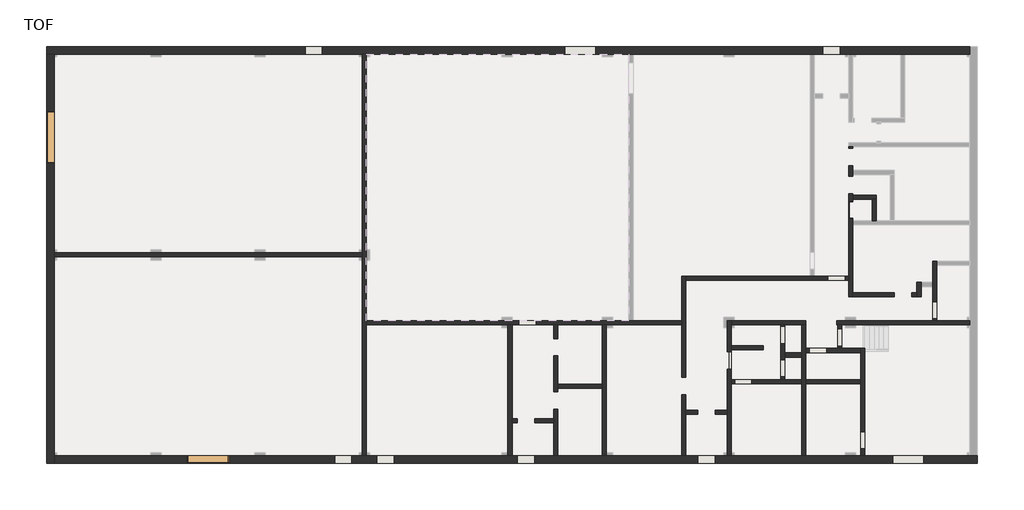
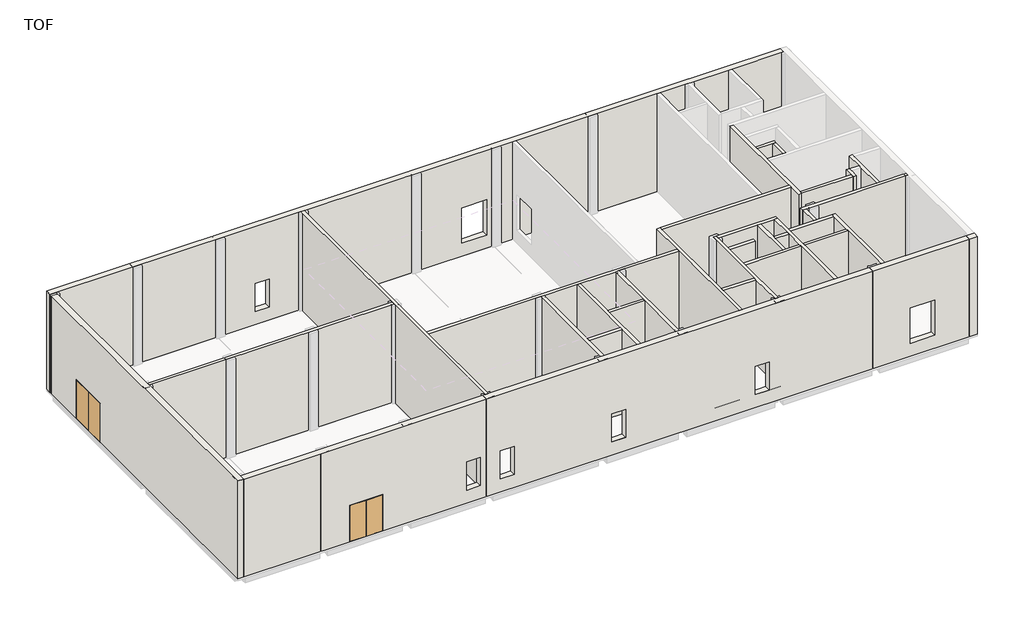
# One storey, part 1 of 3: 31 walls, 3 doors.
# Revit data of these elements (continued)
# Grids (mm) (continued)
#   "Y1": line (-3935.398, 24016.521) -> (58968.688, 24016.521)
#   "X1": line (-75.3, 29394.337) -> (-75.3, -4379.638)
#   "X2": line (5924.7, 29394.337) -> (5924.7, -4379.638)
#   "Y3": line (-3935.398, 8416.521) -> (58968.688, 8416.521)
#   "Y4": line (-3935.398, 616.521) -> (58968.688, 616.521)
#   "X3": line (11924.7, 29394.337) -> (11924.7, -4379.638)
#   "X4": line (17924.7, 29394.337) -> (17924.7, -4379.638)
#   "X5": line (26124.7, 29394.337) -> (26124.7, -4379.638)
#   "X6": line (31924.7, 29394.337) -> (31924.7, -4379.638)
#   "X7": line (38924.7, 29394.337) -> (38924.7, -4379.638)
#   "X8": line (45924.7, 29394.337) -> (45924.7, -4379.638)
#   "X9": line (52924.7, 29394.337) -> (52924.7, -4379.638)
#   "X15": line (43724.7, 27041.858) -> (43724.7, 9156.488)
#   "X16": line (36324.7, 27041.858) -> (36324.7, 9156.488)
#   "X17": line (34685.051, 10966.521) -> (55094.626, 10966.521)
#   "X18": line (34685.051, 18666.521) -> (55094.626, 18666.521)
#   "Y2": line (-3935.398, 12316.521) -> (58968.688, 12316.521)
# Type "Double Door_Steel : H_DR_AMB_Double Door_Steel_W3000xH3000"
#   Type Mark = "362"
#   프레임 = ""
#   철물 = ""
#   유리/마감 = ""
#   위치/개소 = ""
#   부호 = "1/SD"
#   문번호 = ""
#   문기호 = "SD"
#   Analytic Construction = "<None>"
#   Height = 3000.000 mm
#   Width = 3000.000 mm
#   Define Thermal Properties by = 1
#   문 틀 = none
#   문 = none
#   Function = (empty or 0)
#   Assembly Code = ""
#   Wall Closure = (empty or 0)
# Type "Double Door_Steel : H_DR_AMB_Double Door_Steel_W2400xH2800"
#   Type Mark = "365"
#   프레임 = ""
#   철물 = ""
#   유리/마감 = ""
#   위치/개소 = ""
#   부호 = "1/SD"
#   문번호 = ""
#   문기호 = "SD"
#   Analytic Construction = "<None>"
#   Height = 2800.000 mm
#   Width = 2400.000 mm
#   Define Thermal Properties by = 1
#   문 틀 = none
#   문 = none
#   Function = (empty or 0)
#   Assembly Code = ""
#   Wall Closure = (empty or 0)
# Type "Double Door_Steel : H_DR_AMB_Double Door_Steel_W1000xH2150"
#   Type Mark = "366"
#   프레임 = ""
#   철물 = ""
#   유리/마감 = ""
#   위치/개소 = ""
#   부호 = "1/SD"
#   문번호 = ""
#   문기호 = "SD"
#   Analytic Construction = "<None>"
#   Height = 2150.000 mm
#   Width = 1000.000 mm
#   Define Thermal Properties by = 1
#   문 틀 = none
#   문 = none
#   Function = (empty or 0)
#   Assembly Code = ""
#   Wall Closure = (empty or 0)
# Type "H_WA_AMW_Brick Wall_Ext (0.5B_50_1.0B / Emulsion)"
#   Type Comments = ""
#   Layers, outside or top first: 0.000 mm no material (function 100); 20.000 mm no material (function 2); 115.000 mm no material (function 1); 50.000 mm no material (function 3); 0.000 mm no material (function 100); 230.000 mm no material (function 1); 15.000 mm no material (function 2); 0.000 mm no material (function 100); 0.000 mm no material (function 100)
# Type "H_WA_AMW_Block Wall_Int_T200 (Both Plaster_Emulsion)"
#   Type Comments = ""
#   Layers, outside or top first: 0.000 mm no material (function 100); 12.000 mm no material (function 2); 200.000 mm no material (function 1); 12.000 mm no material (function 2); 10.000 mm no material (function 5)
# Element 1 (IfcDoor, "Double Door_Steel : H_DR_AMB_Double Door_Steel_W3000xH3000")
#   Phase Created = New Construction
# Element 2 (IfcDoor, "Double Door_Steel : H_DR_AMB_Double Door_Steel_W2400xH2800")
#   Phase Created = New Construction
# Element 3 (IfcDoor, "Double Door_Steel : H_DR_AMB_Double Door_Steel_W1000xH2150")
#   Phase Created = New Construction
# Element 4 (IfcWall, "H_WA_AMW_Brick Wall_Ext (0.5B_50_1.0B / Emulsion)")
#   Mark = "EW1"
#   Wall Loca = "EXT"
#   Wall Style Name = "Concrete Wall+Insulation+Gypsum Board"
#   Wall Finish-In = "Acrylic Emulsion Paint on Gypsum Board"
#   Wall Base Material-2 = "Glass Wool (Fiberglass)"
#   Wall Base Material-3 = "Concrete Wall"
#   Wall Finish-Ex = "Acrylic Emulsion Paint on Fair Faced Concrete"
#   Top Offset = 0.000 mm
#   Base Offset = 0.000 mm
#   wall height = 7500.000 mm
#   Wall Style No = EW51-1
#   Phase Created = New Construction
#   Base Constraint = TOF
#   Top Constraint = TOC
#   Materials on its faces: "Default Wall"
# Element 5 (IfcWall, "H_WA_AMW_Brick Wall_Ext (0.5B_50_1.0B / Emulsion)")
#   Mark = "EW2"
#   Wall Loca = "EXT"
#   Wall Style Name = "Concrete Wall+Insulation+Gypsum Board"
#   Wall Finish-In = "Acrylic Emulsion Paint on Gypsum Board"
#   Wall Base Material-2 = "Glass Wool (Fiberglass)"
#   Wall Base Material-3 = "Concrete Wall"
#   Wall Finish-Ex = "Acrylic Emulsion Paint on Fair Faced Concrete"
#   Top Offset = 0.000 mm
#   Base Offset = 0.000 mm
#   wall height = 7500.000 mm
#   Wall Style No = EW51-1
#   Phase Created = New Construction
#   Base Constraint = TOF
#   Top Constraint = TOC
#   Materials on its faces: "Default Wall"
# Element 6 (IfcWall, "H_WA_AMW_Brick Wall_Ext (0.5B_50_1.0B / Emulsion)")
#   Mark = "EW3"
#   Wall Loca = "EXT"
#   Wall Style Name = "Concrete Wall+Insulation+Gypsum Board"
#   Wall Finish-In = "Acrylic Emulsion Paint on Gypsum Board"
#   Wall Base Material-2 = "Glass Wool (Fiberglass)"
#   Wall Base Material-3 = "Concrete Wall"
#   Wall Finish-Ex = "Acrylic Emulsion Paint on Fair Faced Concrete"
#   Top Offset = 0.000 mm
#   Base Offset = 0.000 mm
#   wall height = 7500.000 mm
#   Wall Style No = EW51-1
#   Phase Created = New Construction
#   Base Constraint = TOF
#   Top Constraint = TOC
#   Materials on its faces: "Default Wall"
# Element 7 (IfcWall, "H_WA_AMW_Block Wall_Int_T200 (Both Plaster_Emulsion)")
#   Mark = "W1"
#   Wall Loca = "INT"
#   Wall Style Name = "Block Wall"
#   Wall Ref. = ""
#   Wall Finish-In = "Acrylic Emulsion Paint on Cement Plaster"
#   Wall Base Material-1 = "Concrete Block"
#   Wall Base Material-2 = ""
#   Wall Base Material-3 = ""
#   Wall Finish-Ex = "Acrylic Emulsion Paint on Cement Plaster"
#   Top Offset = 0.000 mm
#   Base Offset = 0.000 mm
#   wall height = 7500.000 mm
#   Wall Style No = IW21
#   Phase Created = New Construction
#   Base Constraint = TOF
#   Top Constraint = TOC
#   Materials on its faces: "Default Wall"
# Element 8 (IfcWall, "H_WA_AMW_Block Wall_Int_T200 (Both Plaster_Emulsion)")
#   Mark = "W2"
#   Wall Loca = "INT"
#   Wall Style Name = "Block Wall"
#   Wall Ref. = ""
#   Wall Finish-In = "Acrylic Emulsion Paint on Cement Plaster"
#   Wall Base Material-1 = "Concrete Block"
#   Wall Base Material-2 = ""
#   Wall Base Material-3 = ""
#   Wall Finish-Ex = "Acrylic Emulsion Paint on Cement Plaster"
#   Top Offset = 0.000 mm
#   Base Offset = 0.000 mm
#   wall height = 7500.000 mm
#   Wall Style No = IW21
#   Phase Created = New Construction
#   Base Constraint = TOF
#   Top Constraint = TOC
#   Materials on its faces: "Default Wall"
# Element 9 (IfcWall, "H_WA_AMW_Block Wall_Int_T200 (Both Plaster_Emulsion)")
#   Mark = "W4"
#   Wall Loca = "INT"
#   Wall Style Name = "Block Wall"
#   Wall Ref. = ""
#   Wall Finish-In = "Acrylic Emulsion Paint on Cement Plaster"
#   Wall Base Material-1 = "Concrete Block"
#   Wall Base Material-2 = ""
#   Wall Base Material-3 = ""
#   Wall Finish-Ex = "Acrylic Emulsion Paint on Cement Plaster"
#   Top Offset = 0.000 mm
#   Base Offset = 0.000 mm
#   wall height = 7500.000 mm
#   Wall Style No = IW21
#   Phase Created = New Construction
#   Base Constraint = TOF
#   Top Constraint = TOC
#   Materials on its faces: "Default Wall"
# Element 10 (IfcWall, "H_WA_AMW_Block Wall_Int_T200 (Both Plaster_Emulsion)")
#   Mark = "W5"
#   Wall Loca = "INT"
#   Wall Style Name = "Block Wall"
#   Wall Ref. = ""
#   Wall Finish-In = "Acrylic Emulsion Paint on Cement Plaster"
#   Wall Base Material-1 = "Concrete Block"
#   Wall Base Material-2 = ""
#   Wall Base Material-3 = ""
#   Wall Finish-Ex = "Acrylic Emulsion Paint on Cement Plaster"
#   built-in parameter 1001111 = 1000.000 mm
#   Top Offset = 0.000 mm
#   Base Offset = 1000.000 mm
#   wall height = 6500.000 mm
#   Wall Style No = IW21
#   Phase Created = New Construction
#   Base Constraint = TOF
#   Top Constraint = TOC
#   Materials on its faces: "Default Wall"
# Element 11 (IfcWall, "H_WA_AMW_Block Wall_Int_T200 (Both Plaster_Emulsion)")
#   Mark = "W6"
#   Wall Loca = "INT"
#   Wall Style Name = "Block Wall"
#   Wall Ref. = ""
#   Wall Finish-In = "Acrylic Emulsion Paint on Cement Plaster"
#   Wall Base Material-1 = "Concrete Block"
#   Wall Base Material-2 = ""
#   Wall Base Material-3 = ""
#   Wall Finish-Ex = "Acrylic Emulsion Paint on Cement Plaster"
#   Top Offset = 0.000 mm
#   Base Offset = 0.000 mm
#   wall height = 7500.000 mm
#   Wall Style No = IW21
#   Phase Created = New Construction
#   Base Constraint = TOF
#   Top Constraint = TOC
#   Materials on its faces: "Default Wall"
# Element 12 (IfcWall, "H_WA_AMW_Block Wall_Int_T200 (Both Plaster_Emulsion)")
#   Mark = "W10"
#   Wall Loca = "INT"
#   Wall Style Name = "Block Wall"
#   Wall Ref. = ""
#   Wall Finish-In = "Acrylic Emulsion Paint on Cement Plaster"
#   Wall Base Material-1 = "Concrete Block"
#   Wall Base Material-2 = ""
#   Wall Base Material-3 = ""
#   Wall Finish-Ex = "Acrylic Emulsion Paint on Cement Plaster"
#   built-in parameter 1001111 = 1000.000 mm
#   Top Offset = 0.000 mm
#   Base Offset = 1000.000 mm
#   wall height = 6500.000 mm
#   Wall Style No = IW21
#   Phase Created = New Construction
#   Base Constraint = TOF
#   Top Constraint = TOC
#   Materials on its faces: "Default Wall"
# Element 13 (IfcWall, "H_WA_AMW_Block Wall_Int_T200 (Both Plaster_Emulsion)")
#   Mark = "W11"
#   Wall Loca = "INT"
#   Wall Style Name = "Block Wall"
#   Wall Ref. = ""
#   Wall Finish-In = "Acrylic Emulsion Paint on Cement Plaster"
#   Wall Base Material-1 = "Concrete Block"
#   Wall Base Material-2 = ""
#   Wall Base Material-3 = ""
#   Wall Finish-Ex = "Acrylic Emulsion Paint on Cement Plaster"
#   Top Offset = 0.000 mm
#   Base Offset = 0.000 mm
#   wall height = 7500.000 mm
#   Wall Style No = IW21
#   Phase Created = New Construction
#   Base Constraint = TOF
#   Top Constraint = TOC
#   Materials on its faces: "Default Wall"
# Element 14 (IfcWall, "H_WA_AMW_Block Wall_Int_T200 (Both Plaster_Emulsion)")
#   Mark = "W13"
#   Wall Loca = "INT"
#   Wall Style Name = "Block Wall"
#   Wall Ref. = ""
#   Wall Finish-In = "Acrylic Emulsion Paint on Cement Plaster"
#   Wall Base Material-1 = "Concrete Block"
#   Wall Base Material-2 = ""
#   Wall Base Material-3 = ""
#   Wall Finish-Ex = "Acrylic Emulsion Paint on Cement Plaster"
#   built-in parameter 1001111 = 1000.000 mm
#   Top Offset = 0.000 mm
#   Base Offset = 1000.000 mm
#   wall height = 6500.000 mm
#   Wall Style No = IW21
#   Phase Created = New Construction
#   Base Constraint = TOF
#   Top Constraint = TOC
#   Materials on its faces: "Default Wall"
# Element 15 (IfcWall, "H_WA_AMW_Block Wall_Int_T200 (Both Plaster_Emulsion)")
#   Mark = "W15"
#   Wall Loca = "INT"
#   Wall Style Name = "Block Wall"
#   Wall Ref. = ""
#   Wall Finish-In = "Acrylic Emulsion Paint on Cement Plaster"
#   Wall Base Material-1 = "Concrete Block"
#   Wall Base Material-2 = ""
#   Wall Base Material-3 = ""
#   Wall Finish-Ex = "Acrylic Emulsion Paint on Cement Plaster"
#   Top Offset = 0.000 mm
#   Base Offset = 0.000 mm
#   wall height = 7500.000 mm
#   Wall Style No = IW21
#   Phase Created = New Construction
#   Base Constraint = TOF
#   Top Constraint = TOC
#   Materials on its faces: "Default Wall"
# Element 16 (IfcWall, "H_WA_AMW_Block Wall_Int_T200 (Both Plaster_Emulsion)")
#   Mark = "W16"
#   Wall Loca = "INT"
#   Wall Style Name = "Block Wall"
#   Wall Ref. = ""
#   Wall Finish-In = "Acrylic Emulsion Paint on Cement Plaster"
#   Wall Base Material-1 = "Concrete Block"
#   Wall Base Material-2 = ""
#   Wall Base Material-3 = ""
#   Wall Finish-Ex = "Acrylic Emulsion Paint on Cement Plaster"
#   Top Offset = 0.000 mm
#   Base Offset = 0.000 mm
#   wall height = 7500.000 mm
#   Wall Style No = IW21
#   Phase Created = New Construction
#   Base Constraint = TOF
#   Top Constraint = TOC
#   Materials on its faces: "Default Wall"
# Element 17 (IfcWall, "H_WA_AMW_Block Wall_Int_T200 (Both Plaster_Emulsion)")
#   Mark = "W17"
#   Wall Loca = "INT"
#   Wall Style Name = "Block Wall"
#   Wall Ref. = ""
#   Wall Finish-In = "Acrylic Emulsion Paint on Cement Plaster"
#   Wall Base Material-1 = "Concrete Block"
#   Wall Base Material-2 = ""
#   Wall Base Material-3 = ""
#   Wall Finish-Ex = "Acrylic Emulsion Paint on Cement Plaster"
#   Top Offset = 0.000 mm
#   Base Offset = 0.000 mm
#   wall height = 7500.000 mm
#   Wall Style No = IW21
#   Phase Created = New Construction
#   Base Constraint = TOF
#   Top Constraint = TOC
#   Materials on its faces: "Default Wall"
# Element 18 (IfcWall, "H_WA_AMW_Block Wall_Int_T200 (Both Plaster_Emulsion)")
#   Mark = "W18"
#   Wall Loca = "INT"
#   Wall Style Name = "Block Wall"
#   Wall Ref. = ""
#   Wall Finish-In = "Acrylic Emulsion Paint on Cement Plaster"
#   Wall Base Material-1 = "Concrete Block"
#   Wall Base Material-2 = ""
#   Wall Base Material-3 = ""
#   Wall Finish-Ex = "Acrylic Emulsion Paint on Cement Plaster"
#   Top Offset = 0.000 mm
#   Base Offset = 0.000 mm
#   wall height = 7500.000 mm
#   Wall Style No = IW21
#   Phase Created = New Construction
#   Base Constraint = TOF
#   Top Constraint = TOC
#   Materials on its faces: "Default Wall"
# Element 19 (IfcWall, "H_WA_AMW_Block Wall_Int_T200 (Both Plaster_Emulsion)")
#   Mark = "W19"
#   Wall Loca = "INT"
#   Wall Style Name = "Block Wall"
#   Wall Ref. = ""
#   Wall Finish-In = "Acrylic Emulsion Paint on Cement Plaster"
#   Wall Base Material-1 = "Concrete Block"
#   Wall Base Material-2 = ""
#   Wall Base Material-3 = ""
#   Wall Finish-Ex = "Acrylic Emulsion Paint on Cement Plaster"
#   Top Offset = 0.000 mm
#   Base Offset = 0.000 mm
#   wall height = 7500.000 mm
#   Wall Style No = IW21
#   Phase Created = New Construction
#   Base Constraint = TOF
#   Top Constraint = TOC
#   Materials on its faces: "Default Wall"
# Element 20 (IfcWall, "H_WA_AMW_Block Wall_Int_T200 (Both Plaster_Emulsion)")
#   Mark = "W20"
#   Wall Loca = "INT"
#   Wall Style Name = "Block Wall"
#   Wall Ref. = ""
#   Wall Finish-In = "Acrylic Emulsion Paint on Cement Plaster"
#   Wall Base Material-1 = "Concrete Block"
#   Wall Base Material-2 = ""
#   Wall Base Material-3 = ""
#   Wall Finish-Ex = "Acrylic Emulsion Paint on Cement Plaster"
#   Top Offset = 0.000 mm
#   Base Offset = 0.000 mm
#   wall height = 7500.000 mm
#   Wall Style No = IW21
#   Phase Created = New Construction
#   Base Constraint = TOF
#   Top Constraint = TOC
#   Materials on its faces: "Default Wall"
# Element 21 (IfcWall, "H_WA_AMW_Block Wall_Int_T200 (Both Plaster_Emulsion)")
#   Mark = "W21"
#   Wall Loca = "INT"
#   Wall Style Name = "Block Wall"
#   Wall Ref. = ""
#   Wall Finish-In = "Acrylic Emulsion Paint on Cement Plaster"
#   Wall Base Material-1 = "Concrete Block"
#   Wall Base Material-2 = ""
#   Wall Base Material-3 = ""
#   Wall Finish-Ex = "Acrylic Emulsion Paint on Cement Plaster"
#   Top Offset = 0.000 mm
#   Base Offset = 0.000 mm
#   wall height = 7500.000 mm
#   Wall Style No = IW21
#   Phase Created = New Construction
#   Base Constraint = TOF
#   Top Constraint = TOC
#   Materials on its faces: "Default Wall"
# Element 22 (IfcWall, "H_WA_AMW_Block Wall_Int_T200 (Both Plaster_Emulsion)")
#   Mark = "W22"
#   Wall Loca = "INT"
#   Wall Style Name = "Block Wall"
#   Wall Ref. = ""
#   Wall Finish-In = "Acrylic Emulsion Paint on Cement Plaster"
#   Wall Base Material-1 = "Concrete Block"
#   Wall Base Material-2 = ""
#   Wall Base Material-3 = ""
#   Wall Finish-Ex = "Acrylic Emulsion Paint on Cement Plaster"
#   Top Offset = 0.000 mm
#   Base Offset = 0.000 mm
#   wall height = 7500.000 mm
#   Wall Style No = IW21
#   Phase Created = New Construction
#   Base Constraint = TOF
#   Top Constraint = TOC
#   Materials on its faces: "Default Wall"
# Element 23 (IfcWall, "H_WA_AMW_Block Wall_Int_T200 (Both Plaster_Emulsion)")
#   Mark = "W23"
#   Wall Loca = "INT"
#   Wall Style Name = "Block Wall"
#   Wall Ref. = ""
#   Wall Finish-In = "Acrylic Emulsion Paint on Cement Plaster"
#   Wall Base Material-1 = "Concrete Block"
#   Wall Base Material-2 = ""
#   Wall Base Material-3 = ""
#   Wall Finish-Ex = "Acrylic Emulsion Paint on Cement Plaster"
#   Top Offset = 0.000 mm
#   Base Offset = 0.000 mm
#   wall height = 7500.000 mm
#   Wall Style No = IW21
#   Phase Created = New Construction
#   Base Constraint = TOF
#   Top Constraint = TOC
#   Materials on its faces: "Default Wall"
# Element 24 (IfcWall, "H_WA_AMW_Block Wall_Int_T200 (Both Plaster_Emulsion)")
#   Mark = "W24"
#   Wall Loca = "INT"
#   Wall Style Name = "Block Wall"
#   Wall Ref. = ""
#   Wall Finish-In = "Acrylic Emulsion Paint on Cement Plaster"
#   Wall Base Material-1 = "Concrete Block"
#   Wall Base Material-2 = ""
#   Wall Base Material-3 = ""
#   Wall Finish-Ex = "Acrylic Emulsion Paint on Cement Plaster"
#   Top Offset = 0.000 mm
#   Base Offset = 0.000 mm
#   wall height = 7500.000 mm
#   Wall Style No = IW21
#   Phase Created = New Construction
#   Base Constraint = TOF
#   Top Constraint = TOC
#   Materials on its faces: "Default Wall"
# Element 25 (IfcWall, "H_WA_AMW_Block Wall_Int_T200 (Both Plaster_Emulsion)")
#   Mark = "W25"
#   Wall Loca = "INT"
#   Wall Style Name = "Block Wall"
#   Wall Ref. = ""
#   Wall Finish-In = "Acrylic Emulsion Paint on Cement Plaster"
#   Wall Base Material-1 = "Concrete Block"
#   Wall Base Material-2 = ""
#   Wall Base Material-3 = ""
#   Wall Finish-Ex = "Acrylic Emulsion Paint on Cement Plaster"
#   built-in parameter 1001111 = 1000.000 mm
#   Top Offset = 0.000 mm
#   Base Offset = 1000.000 mm
#   wall height = 6500.000 mm
#   Wall Style No = IW21
#   Phase Created = New Construction
#   Base Constraint = TOF
#   Top Constraint = TOC
#   Materials on its faces: "Default Wall"
# Element 26 (IfcWall, "H_WA_AMW_Block Wall_Int_T200 (Both Plaster_Emulsion)")
#   Mark = "W26"
#   Wall Loca = "INT"
#   Wall Style Name = "Block Wall"
#   Wall Ref. = ""
#   Wall Finish-In = "Acrylic Emulsion Paint on Cement Plaster"
#   Wall Base Material-1 = "Concrete Block"
#   Wall Base Material-2 = ""
#   Wall Base Material-3 = ""
#   Wall Finish-Ex = "Acrylic Emulsion Paint on Cement Plaster"
#   built-in parameter 1001111 = 1000.000 mm
#   Top Offset = 0.000 mm
#   Base Offset = 1000.000 mm
#   wall height = 6500.000 mm
#   Wall Style No = IW21
#   Phase Created = New Construction
#   Base Constraint = TOF
#   Top Constraint = TOC
#   Materials on its faces: "Default Wall"
# Element 27 (IfcWall, "H_WA_AMW_Block Wall_Int_T200 (Both Plaster_Emulsion)")
#   Mark = "W27"
#   Wall Loca = "INT"
#   Wall Style Name = "Block Wall"
#   Wall Ref. = ""
#   Wall Finish-In = "Acrylic Emulsion Paint on Cement Plaster"
#   Wall Base Material-1 = "Concrete Block"
#   Wall Base Material-2 = ""
#   Wall Base Material-3 = ""
#   Wall Finish-Ex = "Acrylic Emulsion Paint on Cement Plaster"
#   Top Offset = 0.000 mm
#   Base Offset = 0.000 mm
#   wall height = 7500.000 mm
#   Wall Style No = IW21
#   Phase Created = New Construction
#   Base Constraint = TOF
#   Top Constraint = TOC
#   Materials on its faces: "Default Wall"
# Element 28 (IfcWall, "H_WA_AMW_Block Wall_Int_T200 (Both Plaster_Emulsion)")
#   Mark = "W28"
#   Wall Loca = "INT"
#   Wall Style Name = "Block Wall"
#   Wall Ref. = ""
#   Wall Finish-In = "Acrylic Emulsion Paint on Cement Plaster"
#   Wall Base Material-1 = "Concrete Block"
#   Wall Base Material-2 = ""
#   Wall Base Material-3 = ""
#   Wall Finish-Ex = "Acrylic Emulsion Paint on Cement Plaster"
#   built-in parameter 1001111 = 1000.000 mm
#   Top Offset = 0.000 mm
#   Base Offset = 1000.000 mm
#   wall height = 6500.000 mm
#   Wall Style No = IW21
#   Phase Created = New Construction
#   Base Constraint = TOF
#   Top Constraint = TOC
#   Materials on its faces: "Default Wall"
# Element 29 (IfcWall, "H_WA_AMW_Block Wall_Int_T200 (Both Plaster_Emulsion)")
#   Mark = "W29"
#   Wall Loca = "INT"
#   Wall Style Name = "Block Wall"
#   Wall Ref. = ""
#   Wall Finish-In = "Acrylic Emulsion Paint on Cement Plaster"
#   Wall Base Material-1 = "Concrete Block"
#   Wall Base Material-2 = ""
#   Wall Base Material-3 = ""
#   Wall Finish-Ex = "Acrylic Emulsion Paint on Cement Plaster"
#   built-in parameter 1001111 = 1000.000 mm
#   Top Offset = 0.000 mm
#   Base Offset = 1000.000 mm
#   wall height = 6500.000 mm
#   Wall Style No = IW21
#   Phase Created = New Construction
#   Base Constraint = TOF
#   Top Constraint = TOC
#   Materials on its faces: "Default Wall"
# Element 30 (IfcWall, "H_WA_AMW_Block Wall_Int_T200 (Both Plaster_Emulsion)")
#   Mark = "W31"
#   Wall Loca = "INT"
#   Wall Style Name = "Block Wall"
#   Wall Ref. = ""
#   Wall Finish-In = "Acrylic Emulsion Paint on Cement Plaster"
#   Wall Base Material-1 = "Concrete Block"
#   Wall Base Material-2 = ""
#   Wall Base Material-3 = ""
#   Wall Finish-Ex = "Acrylic Emulsion Paint on Cement Plaster"
#   built-in parameter 1001111 = 1000.000 mm
#   Top Offset = 0.000 mm
#   Base Offset = 1000.000 mm
#   wall height = 6500.000 mm
#   Wall Style No = IW21
#   Phase Created = New Construction
#   Base Constraint = TOF
#   Top Constraint = TOC
#   Materials on its faces: "Default Wall"
# Element 31 (IfcWall, "H_WA_AMW_Block Wall_Int_T200 (Both Plaster_Emulsion)")
#   Mark = "W34"
#   Wall Loca = "INT"
#   Wall Style Name = "Block Wall"
#   Wall Ref. = ""
#   Wall Finish-In = "Acrylic Emulsion Paint on Cement Plaster"
#   Wall Base Material-1 = "Concrete Block"
#   Wall Base Material-2 = ""
#   Wall Base Material-3 = ""
#   Wall Finish-Ex = "Acrylic Emulsion Paint on Cement Plaster"
#   built-in parameter 1001111 = 1000.000 mm
#   Top Offset = 0.000 mm
#   Base Offset = 1000.000 mm
#   wall height = 6500.000 mm
#   Wall Style No = IW21
#   Phase Created = New Construction
#   Base Constraint = TOF
#   Top Constraint = TOC
#   Materials on its faces: "Default Wall"
# Element 32 (IfcWall, "H_WA_AMW_Block Wall_Int_T200 (Both Plaster_Emulsion)")
#   Mark = "W39"
#   Wall Loca = "INT"
#   Wall Style Name = "Block Wall"
#   Wall Ref. = ""
#   Wall Finish-In = "Acrylic Emulsion Paint on Cement Plaster"
#   Wall Base Material-1 = "Concrete Block"
#   Wall Base Material-2 = ""
#   Wall Base Material-3 = ""
#   Wall Finish-Ex = "Acrylic Emulsion Paint on Cement Plaster"
#   built-in parameter 1001111 = 1000.000 mm
#   Top Offset = 0.000 mm
#   Base Offset = 1000.000 mm
#   wall height = 6500.000 mm
#   Wall Style No = IW21
#   Phase Created = New Construction
#   Base Constraint = TOF
#   Top Constraint = TOC
#   Materials on its faces: "Default Wall"
# Element 33 (IfcWall, "H_WA_AMW_Block Wall_Int_T200 (Both Plaster_Emulsion)")
#   Mark = "W40"
#   Wall Loca = "INT"
#   Wall Style Name = "Block Wall"
#   Wall Ref. = ""
#   Wall Finish-In = "Acrylic Emulsion Paint on Cement Plaster"
#   Wall Base Material-1 = "Concrete Block"
#   Wall Base Material-2 = ""
#   Wall Base Material-3 = ""
#   Wall Finish-Ex = "Acrylic Emulsion Paint on Cement Plaster"
#   built-in parameter 1001111 = 1000.000 mm
#   Top Offset = 0.000 mm
#   Base Offset = 1000.000 mm
#   wall height = 6500.000 mm
#   Wall Style No = IW21
#   Phase Created = New Construction
#   Base Constraint = TOF
#   Top Constraint = TOC
#   Materials on its faces: "Default Wall"
# Element 34 (IfcWall, "H_WA_AMW_Block Wall_Int_T200 (Both Plaster_Emulsion)")
#   Mark = "W41"
#   Wall Loca = "INT"
#   Wall Style Name = "Block Wall"
#   Wall Ref. = ""
#   Wall Finish-In = "Acrylic Emulsion Paint on Cement Plaster"
#   Wall Base Material-1 = "Concrete Block"
#   Wall Base Material-2 = ""
#   Wall Base Material-3 = ""
#   Wall Finish-Ex = "Acrylic Emulsion Paint on Cement Plaster"
#   Top Offset = 0.000 mm
#   Base Offset = 0.000 mm
#   wall height = 7500.000 mm
#   Wall Style No = IW21
#   Phase Created = New Construction
#   Base Constraint = TOF
#   Top Constraint = TOC
#   Materials on its faces: "Default Wall"
# Materials
#   "Default Wall": class "Miscellaneous", colour RGB 80 80 80, transparency 0
